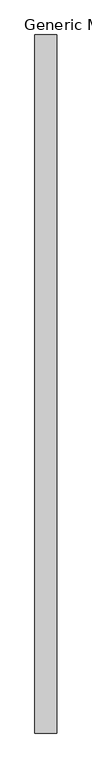
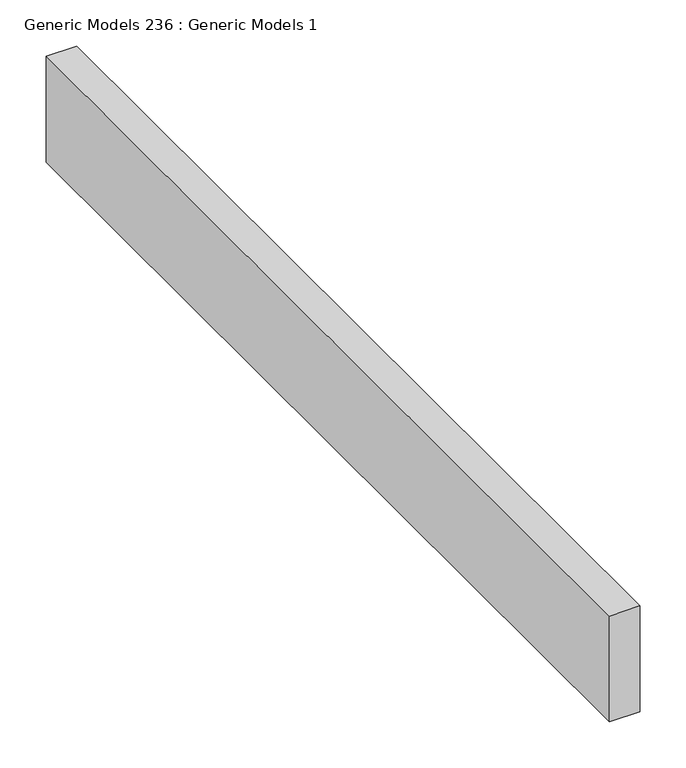
"""IFC4 building model written with IfcOpenShell, lengths in millimetres: proxy geometry, Generic Models 236 : Generic Models 1."""

from ifc_helpers import new_model, si_unit, frame, origin, place, context, project, spatial, polyline, outline, extrude, source, transform, mapped, element, save


def generic_models_236_generic_models_1_f8917e71(model_context):
    return source(origin(), model_context, "Body", "SweptSolid", [
        extrude(outline(polyline([(48507.65, 0.0), (48469.55, 0.0), (48469.55, 1219.2), (48507.65, 1219.2), (48507.65, 0.0)])), frame((0.0, 0.0, 5507.83125), z_axis=(0.0, 0.0, 1.0), x_axis=(1.0, 0.0, 0.0)), (0.0, 0.0, 1.0), 139.7),
    ])


if __name__ == "__main__":
    model = new_model("IFC4")
    model_context = context("Model", 3, world=origin())
    ifc_project = project(units=[si_unit("LENGTHUNIT", "METRE", prefix="MILLI")], contexts=[model_context])
    site = spatial("IfcSite", under=ifc_project)
    building = spatial("IfcBuilding", under=site)
    placement = place(None, origin())
    generic_models_236_generic_models_1_shape = generic_models_236_generic_models_1_f8917e71(model_context)
    element("IfcBuildingElementProxy", 1, Name="Generic Models 236 : Generic Models 1", ObjectType="Generic Models 236 : Generic Models 1", at=placement, inside=building, context=model_context, shape_type="MappedRepresentation", body=[
        mapped(generic_models_236_generic_models_1_shape, transform((0.0, 0.0, 0.0), x_axis=(1.0, 0.0, 0.0), y_axis=(0.0, 1.0, 0.0), z_axis=(0.0, 0.0, 1.0))),
    ])
    save(model, "model.ifc")

# Revit data of these elements
# Element 1 (IfcBuildingElementProxy, "Generic Models 236 : Generic Models 1")
#   Materials on its faces: "EXISTING RIM BOARD OR JOIST"
# Materials
#   "EXISTING RIM BOARD OR JOIST": class "Wood", colour RGB 234 198 147, transparency 0, Description = "Pinus Echinata", Cost = 0
